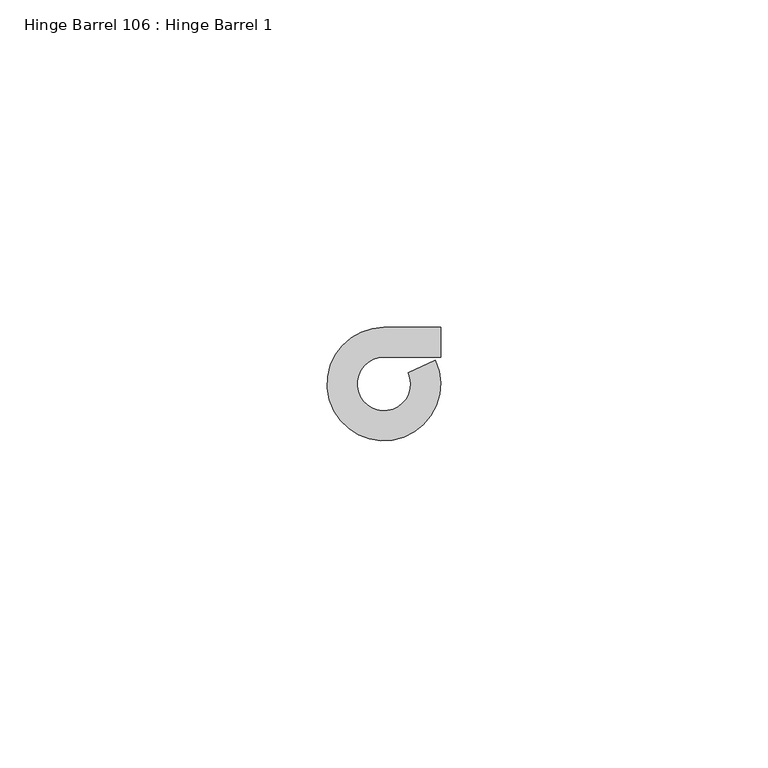
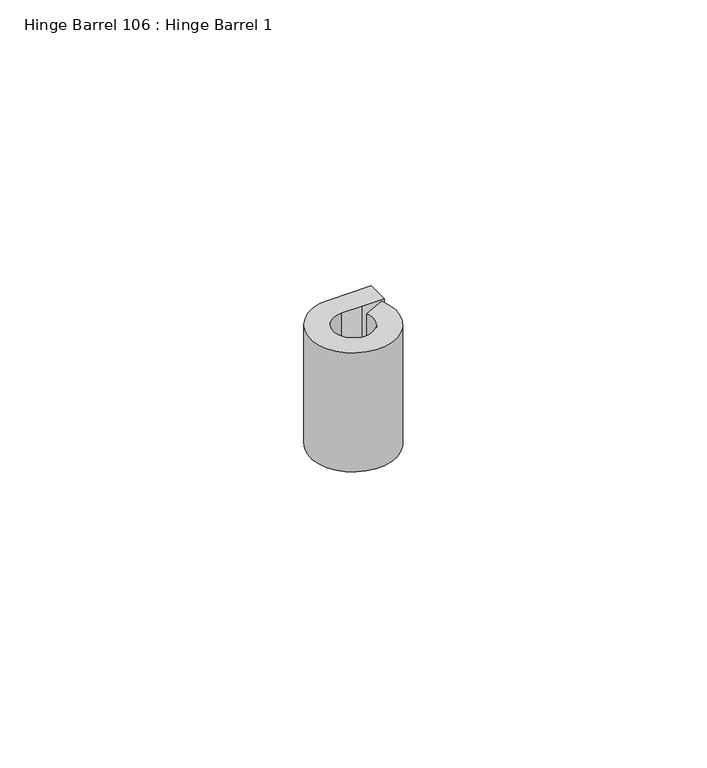
"""IFC4 building model written with IfcOpenShell, lengths in millimetres: proxy geometry, Hinge Barrel 106 : Hinge Barrel 1."""

from ifc_helpers import new_model, si_unit, point, frame, frame_2d, origin, place, context, project, spatial, polyline, circle_curve, trimmed, segment, composite_curve, outline, extrude, source, transform, mapped, element, save


def hinge_barrel_106_hinge_barrel_1_1aaac7a2(model_context):
    return source(origin(), model_context, "Body", "SweptSolid", [
        extrude(outline(composite_curve([segment(polyline([(587323.2214739, -533980.5883841), (587319.1320739, -533980.5883841)]), True, "CONTINUOUS"), segment(trimmed(circle_curve(frame_2d((587319.1320739, -533984.6777841)), 4.0894), [point((587319.1320739, -533980.5883841))], [point((587322.8436736, -533982.9610371))], True, "CARTESIAN"), True, "CONTINUOUS"), segment(polyline([(587322.8436736, -533982.9610371), (587326.986084, -533981.0450249)]), True, "CONTINUOUS"), segment(trimmed(circle_curve(frame_2d((587319.1320739, -533984.6777841)), 8.6534625), [point((587326.986084, -533981.0450249))], [point((587319.1320739, -533976.0243216))], False, "CARTESIAN"), True, "CONTINUOUS"), segment(polyline([(587319.1320739, -533976.0243216), (587327.7934739, -533976.0243216), (587327.7934739, -533980.5883841), (587323.2214739, -533980.5883841)]), True, "CONTINUOUS")], self_intersect=False)), frame((0.0, 0.0, 1225.55), z_axis=(0.0, 0.0, 1.0), x_axis=(1.0, 0.0, 0.0)), (0.0, 0.0, 1.0), 25.4),
    ])


if __name__ == "__main__":
    model = new_model("IFC4")
    model_context = context("Model", 3, world=origin())
    ifc_project = project(units=[si_unit("LENGTHUNIT", "METRE", prefix="MILLI")], contexts=[model_context])
    site = spatial("IfcSite", under=ifc_project)
    building = spatial("IfcBuilding", under=site)
    placement = place(None, origin())
    hinge_barrel_106_hinge_barrel_1_shape = hinge_barrel_106_hinge_barrel_1_1aaac7a2(model_context)
    element("IfcBuildingElementProxy", 1, Name="Hinge Barrel 106 : Hinge Barrel 1", ObjectType="Hinge Barrel 106 : Hinge Barrel 1", at=placement, inside=building, context=model_context, shape_type="MappedRepresentation", body=[
        mapped(hinge_barrel_106_hinge_barrel_1_shape, transform((0.0, 0.0, 0.0), x_axis=(1.0, 0.0, 0.0), y_axis=(0.0, 1.0, 0.0), z_axis=(0.0, 0.0, 1.0))),
    ])
    save(model, "model.ifc")

# Revit data of these elements
# Element 1 (IfcBuildingElementProxy, "Hinge Barrel 106 : Hinge Barrel 1")
#   Materials on its faces: "6\"X6\" WELD-ON STL BUTT HINGE"
# Materials
#   "6\"X6\" WELD-ON STL BUTT HINGE": class "Metal", colour RGB 189 187 185, transparency 0, Description = "Carbon steel", Cost = 0
